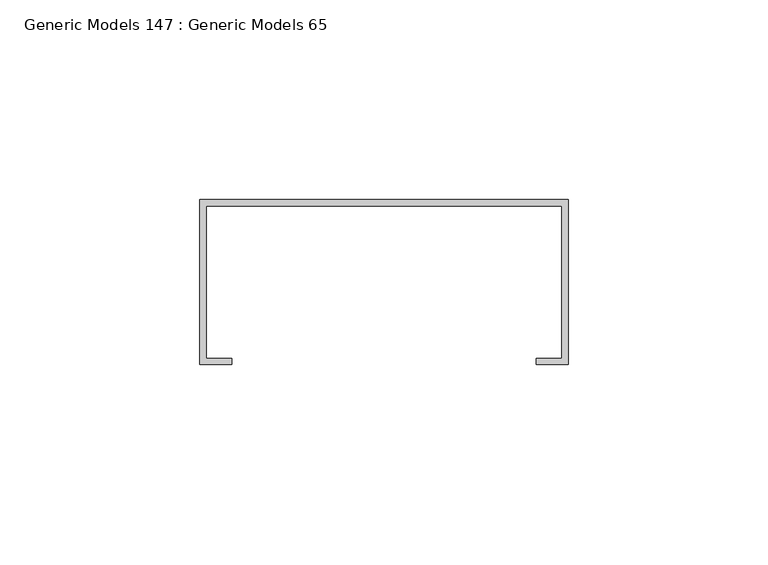
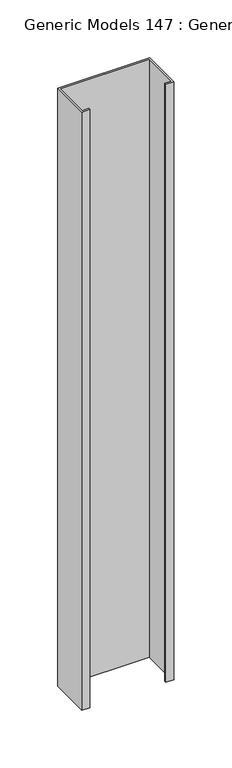
"""IFC4 building model written with IfcOpenShell, lengths in millimetres: proxy geometry, Generic Models 147 : Generic Models 65."""

from ifc_helpers import new_model, si_unit, frame, origin, place, context, project, spatial, polyline, outline, extrude, source, transform, mapped, element, save


def generic_models_147_generic_models_65_fc30ab23(model_context):
    return source(origin(), model_context, "Body", "SweptSolid", [
        extrude(outline(polyline([(48062.9985531, 630.2375), (48155.0735531, 630.2375), (48155.0735531, 588.9625), (48147.1360531, 588.9625), (48147.1360531, 590.55), (48153.4860531, 590.55), (48153.4860531, 628.65), (48064.5860531, 628.65), (48064.5860531, 590.55), (48070.9360531, 590.55), (48070.9360531, 588.9625), (48062.9985531, 588.9625), (48062.9985531, 630.2375)])), frame((0.0, 0.0, 1598.2598705), z_axis=(0.0, 0.0, 1.0), x_axis=(1.0, 0.0, 0.0)), (0.0, 0.0, 1.0), 631.6265625),
    ])


if __name__ == "__main__":
    model = new_model("IFC4")
    model_context = context("Model", 3, world=origin())
    ifc_project = project(units=[si_unit("LENGTHUNIT", "METRE", prefix="MILLI")], contexts=[model_context])
    site = spatial("IfcSite", under=ifc_project)
    building = spatial("IfcBuilding", under=site)
    placement = place(None, origin())
    generic_models_147_generic_models_65_shape = generic_models_147_generic_models_65_fc30ab23(model_context)
    element("IfcBuildingElementProxy", 1, Name="Generic Models 147 : Generic Models 65", ObjectType="Generic Models 147 : Generic Models 65", at=placement, inside=building, context=model_context, shape_type="MappedRepresentation", body=[
        mapped(generic_models_147_generic_models_65_shape, transform((0.0, 0.0, 0.0), x_axis=(1.0, 0.0, 0.0), y_axis=(0.0, 1.0, 0.0), z_axis=(0.0, 0.0, 1.0))),
    ])
    save(model, "model.ifc")

# Revit data of these elements
# Element 1 (IfcBuildingElementProxy, "Generic Models 147 : Generic Models 65")
#   Materials on its faces: "METAL STUD (16\" O.C.)"
# Materials
#   "METAL STUD (16\" O.C.)": class "Unassigned", colour RGB 210 209 208, transparency 0, Keynote = "M05121300.02", Cost = 0
